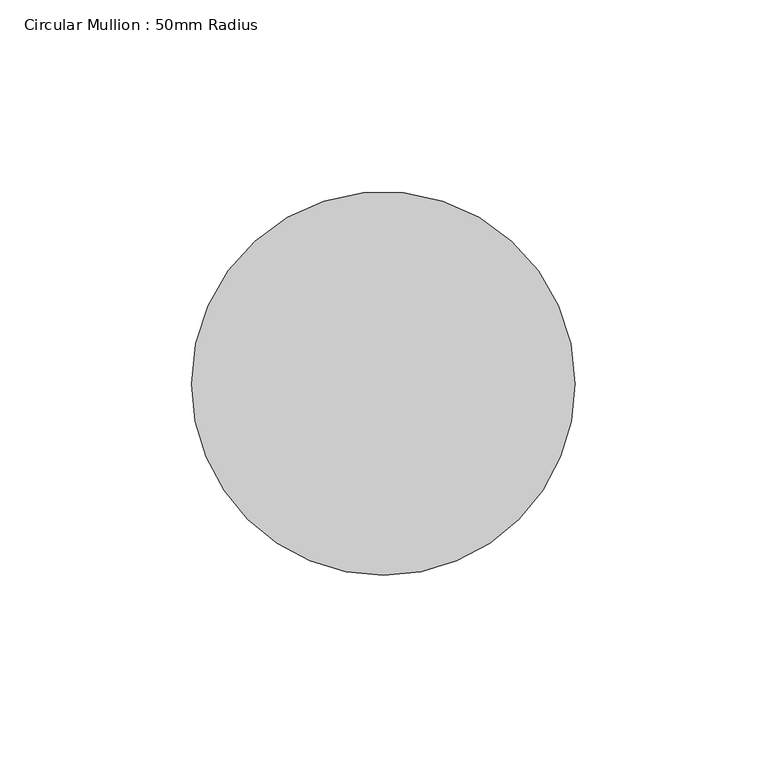
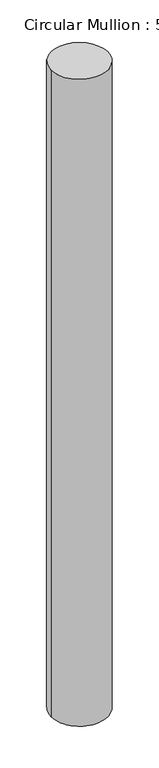
"""IFC4 building model written with IfcOpenShell, lengths in millimetres: member geometry, Circular Mullion : 50mm Radius."""

from ifc_helpers import new_model, si_unit, frame, origin, place, context, project, spatial, ellipse_curve, source, transform, mapped, element, save
from ifc_brep_helpers import plane_surface, cylinder_surface, advanced_brep


def circular_mullion_50mm_radius_4c91948a(model_context):
    return source(origin(), model_context, "Body", "AdvancedBrep", [
        advanced_brep(
        [(-100.0, 0.0, 0.7030841), (0.0, 0.0, 0.0), (0.0, 0.0, -1202.0418058), (-100.0, 0.0, -1202.7151335)],
        [
            (0, 1, ellipse_curve(frame((-50.0, 0.0, 0.3515421), z_axis=(-0.007030065157579015, -0.013090725362707892, -0.9998895994525389), x_axis=(-0.4730671340544569, -0.8809010715005751, 0.014858967213143101)), 50.0055206, 50.0)),
            (1, 2),
            (2, 3, ellipse_curve(frame((-50.0, 0.0, -1202.3784696), z_axis=(-0.00673259496136123, -0.012536804374069075, 0.9998987452243215), x_axis=(0.4730714610962257, 0.8809091289102724, 0.014230224834035956)), 50.0050633, 50.0)),
            (3, 0),
            (1, 0, ellipse_curve(frame((-50.0, 0.0, 0.3515421), z_axis=(-0.007030065157579015, -0.013090725362707892, -0.9998895994525389), x_axis=(-0.4730671340544569, -0.8809010715005751, 0.014858967213143101)), 50.0055206, 50.0)),
            (3, 2, ellipse_curve(frame((-50.0, 0.0, -1202.3784696), z_axis=(-0.00673259496136123, -0.012536804374069075, 0.9998987452243215), x_axis=(0.4730714610962257, 0.8809091289102724, 0.014230224834035956)), 50.0050633, 50.0)),
        ],
        [
            cylinder_surface(frame((-50.0, 0.0, 0.0), z_axis=(0.0, 0.0, 1.0), x_axis=(1.0, 0.0, 0.0)), 50.0),
            plane_surface(frame((-268.5282923, 144.206783, 0.0), z_axis=(0.007030065157579015, 0.013090725362707892, 0.9998895994525389), x_axis=(0.47306713405445516, 0.8809010715005758, -0.014858967213156172))),
            plane_surface(frame((-268.5282923, 144.206783, -1202.0418058), z_axis=(0.00673259496136123, 0.012536804374069075, -0.9998987452243215), x_axis=(0.4730714610962256, 0.8809091289102724, 0.01423022483404335))),
        ],
        [
            (0, [[1, 2, 3, 4]]),
            (0, [[5, -4, 6, -2]]),
            (1, [[-1, -5]]),
            (2, [[-6, -3]]),
        ],
    ),
    ])


if __name__ == "__main__":
    model = new_model("IFC4")
    model_context = context("Model", 3, world=origin())
    ifc_project = project(units=[si_unit("LENGTHUNIT", "METRE", prefix="MILLI")], contexts=[model_context])
    site = spatial("IfcSite", under=ifc_project)
    building = spatial("IfcBuilding", under=site)
    placement = place(None, origin())
    circular_mullion_50mm_radius_shape = circular_mullion_50mm_radius_4c91948a(model_context)
    element("IfcMember", 1, ObjectType="Circular Mullion : 50mm Radius", at=placement, inside=building, context=model_context, shape_type="MappedRepresentation", body=[
        mapped(circular_mullion_50mm_radius_shape, transform((0.0, 0.0, 0.0), x_axis=(1.0, 0.0, 0.0), y_axis=(0.0, 1.0, 0.0), z_axis=(0.0, 0.0, 1.0))),
    ])
    save(model, "model.ifc")

# Revit data of these elements
# Type "Circular Mullion : 50mm Radius"
#   built-in parameter 1007350 = 0.164042 (stored number, unit not read)
# Element 1 (IfcMember, "Circular Mullion : 50mm Radius")
#   Materials on its faces: "Aluminium"
# Materials
#   "Aluminium": class "Metal", colour RGB 247 247 247, transparency 0, Description = "Aluminium 6061", Cost = 0
